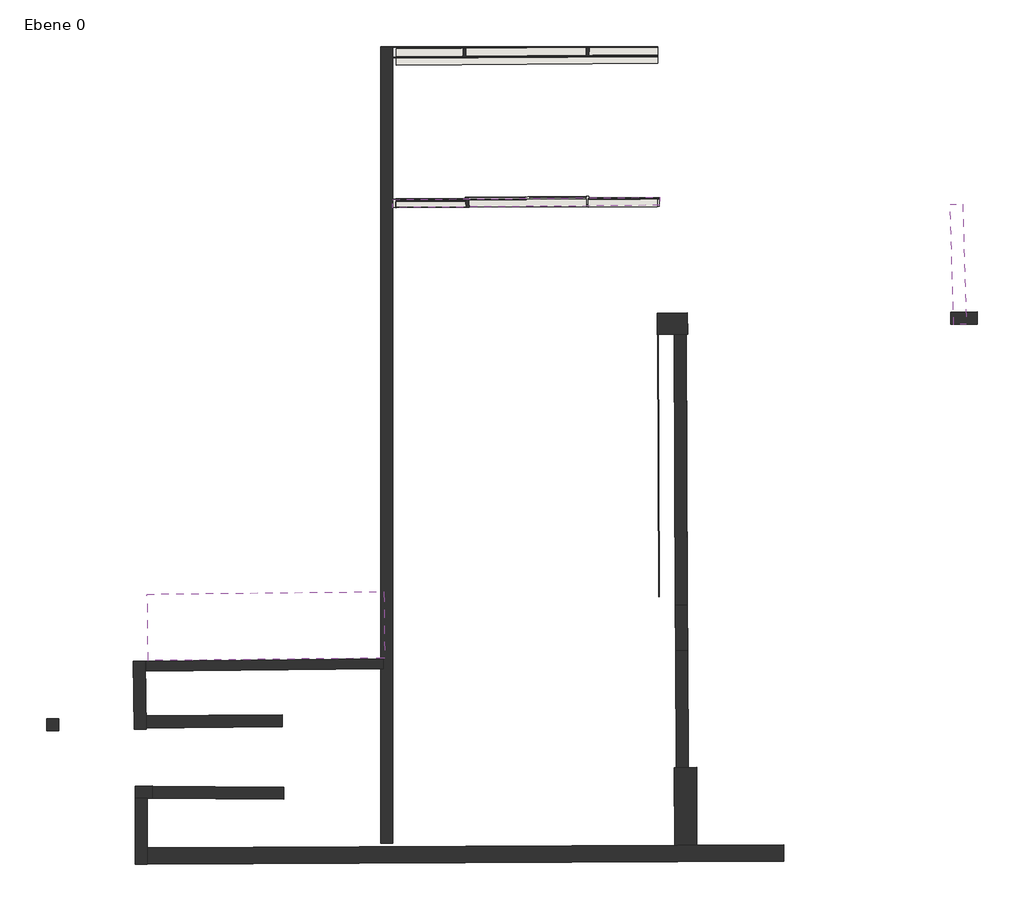
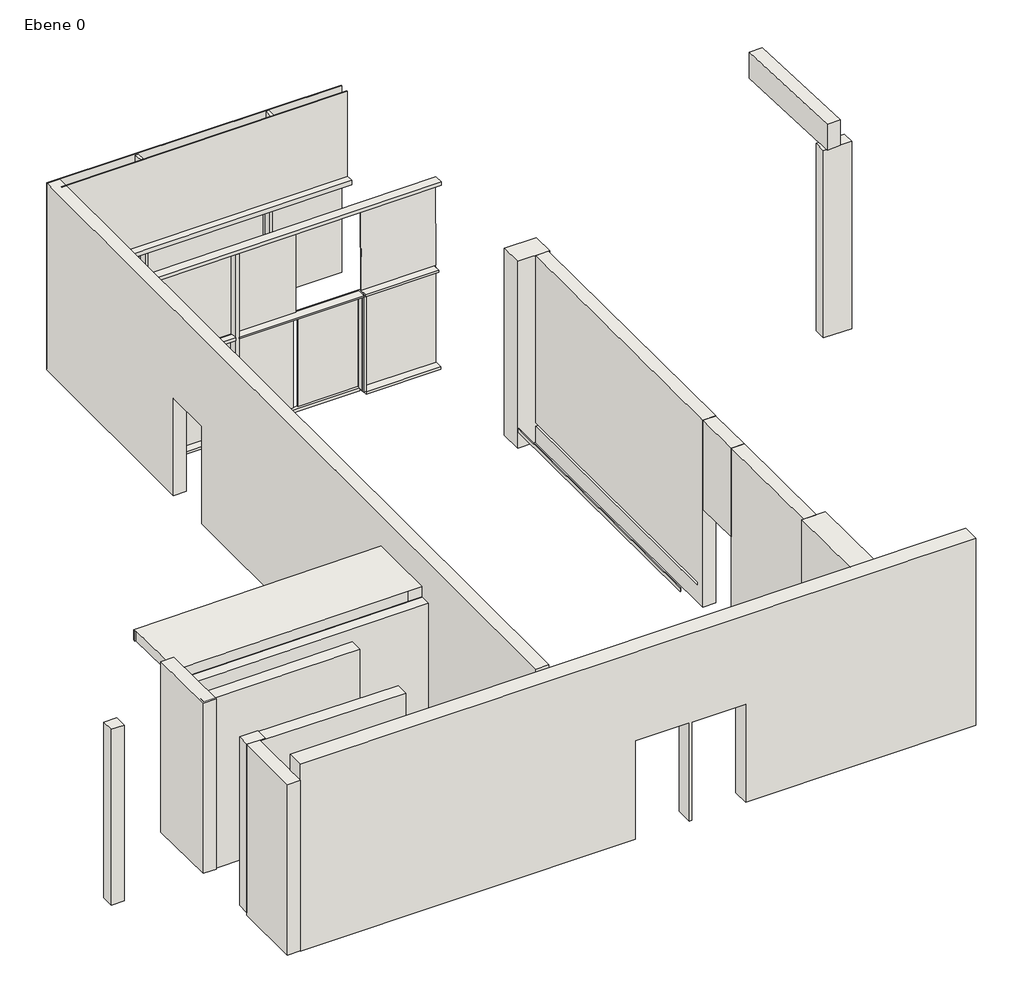
# One storey: 46 walls.
"""IFC4 building model written with IfcOpenShell, lengths in millimetres."""

from ifc_helpers import new_model, si_unit, frame, origin, place, context, project, spatial, polyline, outline, extrude, faceted_brep, element, save

model = new_model("IFC4")

# Units and contexts
model_context = context("Model", 3, world=origin())
ifc_project = project(units=[si_unit("LENGTHUNIT", "METRE", prefix="MILLI")], contexts=[model_context])

# Site, building, storey
site = spatial("IfcSite", under=ifc_project)
building = spatial("IfcBuilding", under=site)
storey = spatial("IfcBuildingStorey", under=building, Name="Ebene 0", Elevation=0.0)

# Walls
placement = place(None, origin())
element("IfcWall", 1, ObjectType="STB 30.0 - Sichtbeton 1", at=placement, inside=storey, context=model_context, shape_type="SweptSolid", body=[
    extrude(outline(polyline([(-8402.8984862, -3386.1116182), (-5023.0576004, -3407.986993), (-5024.9992525, -3707.9807096), (-8404.8401383, -3686.1053348), (-8402.8984862, -3386.1116182)])), frame((0.0, 0.0, -1567.0079424), z_axis=(0.0, 0.0, 1.0), x_axis=(1.0, 0.0, 0.0)), (0.0, 0.0, 1.0), 4193.9637451),
])
element("IfcWall", 2, ObjectType="STB 30.0 - Sichtbeton 1", at=placement, inside=storey, context=model_context, shape_type="SweptSolid", body=[
    extrude(outline(polyline([(-8711.881099, -1641.309095), (-5062.179794, -1608.676683), (-5059.4975656, -1908.6646922), (-8709.1988706, -1941.2971042), (-8711.881099, -1641.309095)])), frame((0.0, 0.0, -1566.6113359), z_axis=(0.0, 0.0, 1.0), x_axis=(1.0, 0.0, 0.0)), (0.0, 0.0, 1.0), 4193.494873),
])
element("IfcWall", 3, ObjectType="STB 30.0 - Sichtbeton 1", at=placement, inside=storey, context=model_context, shape_type="Brep", body=[
    faceted_brep([(-8280.7224922, -3375.8727385, -1505.4189133), (-8707.8712691, -3380.2933626, -1505.4189133), (-8707.8712691, -3380.2933626, 2636.550325), (-8280.7224922, -3375.8727385, 2636.550325), (-8280.7224922, -3375.8727385, -1388.9973215), (-8280.4523049, -3675.8860076, -1505.4189133), (-8280.4523049, -3675.8860076, 2636.550325), (-8407.8712691, -3677.2046848, 2636.550325), (-8707.8712691, -3680.3094278, 2636.550325), (-8707.8712691, -3680.3094278, -1505.4189133)], [[[0, 1, 2, 3, 4]], [[5, 6, 7, 8, 9]], [[1, 0, 5, 9]], [[3, 2, 8, 7, 6]], [[0, 4, 3, 6, 5]], [[2, 1, 9, 8]]]),
])
element("IfcWall", 4, ObjectType="STB 30.0 - Sichtbeton 1", at=placement, inside=storey, context=model_context, shape_type="Brep", body=[
    faceted_brep([(-8407.8712691, -5310.6242916, -1565.0), (-8407.8712691, -3677.2046848, -1565.0), (-8407.8712691, -3677.2046848, 2636.550325), (-8407.8712691, -5310.6242916, 2636.550325), (-8707.8712691, -5312.0476748, -1565.0), (-8707.8712691, -5312.0476748, 2636.550325), (-8707.8712691, -3680.3094278, 2636.550325), (-8707.8712691, -3680.3094278, -1505.4189133), (-8707.8712691, -3680.3094278, -1565.0)], [[[0, 1, 2, 3]], [[4, 5, 6, 7, 8]], [[1, 0, 4, 8]], [[3, 2, 6, 5]], [[2, 1, 8, 7, 6]], [[0, 3, 5, 4]]]),
])
element("IfcWall", 5, ObjectType="STB 30.0 - Sichtbeton 1", at=placement, inside=storey, context=model_context, shape_type="SweptSolid", body=[
    extrude(outline(polyline([(-8454.8872938, -283.8713377), (-8435.0535607, -1969.7388339), (-8735.0328016, -1973.268001), (-8754.8665347, -287.4005048), (-8454.8872938, -283.8713377)])), frame((0.0, 0.0, -1567.5369553), z_axis=(0.0, 0.0, 1.0), x_axis=(1.0, 0.0, 0.0)), (0.0, 0.0, 1.0), 4195.9727783),
])
element("IfcWall", 6, ObjectType="STB 30.0 - Sichtbeton 1", at=placement, inside=storey, context=model_context, shape_type="SweptSolid", body=[
    extrude(outline(polyline([(-10898.8481887, -2010.6735209), (-10902.7495019, -1710.7000992), (-10602.7748702, -1706.7987702), (-10598.873557, -2006.772192), (-10898.8481887, -2010.6735209)])), frame((0.0, 0.0, -1564.2386155), z_axis=(0.0, 0.0, 1.0), x_axis=(1.0, 0.0, 0.0)), (0.0, 0.0, 1.0), 4321.9161377),
])
element("IfcWall", 7, ObjectType="STB 30.0 - Sichtbeton 1", at=placement, inside=storey, context=model_context, shape_type="Brep", body=[
    faceted_brep([(4640.0905057, 7800.3536755, -1082.1717735), (4667.2831216, 1312.227188, -1082.1717735), (4667.2831216, 1312.227188, -1172.1717735), (4640.0905057, 7800.3536755, -1172.1717735), (4640.0905057, 7800.3536755, -1570.8115996), (4668.150891, 1105.1784267, -1570.8115996), (4668.150891, 1105.1784267, 3029.0079909), (4640.0905057, 7800.3536755, 3029.0079909), (4940.0878709, 7801.6110051, -1082.1717735), (4940.0878709, 7801.6110051, 3029.0079909), (4968.1456336, 1107.0614957, 3029.0079909), (4968.1456336, 1107.0614957, -1570.8115996), (4940.0878709, 7801.6110051, -1570.8115996), (4940.0878709, 7801.6110051, -1172.1717735), (4967.2804868, 1313.4845175, -1172.1717735), (4967.2804868, 1313.4845175, -1082.1717735)], [[[0, 1, 2, 3, 4, 5, 6, 7]], [[8, 9, 10, 11, 12, 13, 14, 15]], [[1, 0, 8, 15]], [[2, 1, 15, 14]], [[3, 2, 14, 13]], [[4, 3, 13, 12]], [[5, 4, 12, 11]], [[7, 6, 10, 9]], [[0, 7, 9, 8]], [[6, 5, 11, 10]]]),
])
element("IfcWall", 8, ObjectType="STB 30.0 - Sichtbeton 1", at=placement, inside=storey, context=model_context, shape_type="Brep", body=[
    faceted_brep([(4677.6567247, -31.4843616, 3026.055442), (4668.150891, 1105.1784267, 3026.055442), (4668.150891, 1105.1784267, 833.3), (4668.1769602, 1102.061196, 833.3), (4668.1769602, 1102.061196, 843.3), (4677.6567247, -31.4843616, 843.3), (4968.1456336, 1107.0614956, 3026.055442), (4977.6502256, -29.4528133, 3026.055442), (4977.6502256, -29.4528133, 843.3), (4968.1664699, 1104.5699879, 843.3), (4968.1664699, 1104.5699879, 833.3), (4968.1456336, 1107.0614956, 833.3)], [[[0, 1, 2, 3, 4, 5]], [[6, 7, 8, 9, 10, 11]], [[2, 11, 10, 3]], [[1, 0, 7, 6]], [[2, 1, 6, 11]], [[7, 0, 5, 8]], [[4, 9, 8, 5]], [[9, 4, 3, 10]]]),
])
element("IfcWall", 9, ObjectType="STB 30.0 - Sichtbeton 1", at=placement, inside=storey, context=model_context, shape_type="Brep", body=[
    faceted_brep([(4692.6152809, -2918.6509775, 3026.055442), (4677.6567247, -31.4843616, 3026.055442), (4677.6567247, -31.4843616, 843.3), (4677.6567247, -31.4843616, -1570.8115996), (4677.6744168, -34.8991368, -1570.8115996), (4692.6152809, -2918.6509775, -1570.8115996), (4992.6112545, -2917.0966832, 3026.055442), (4992.6112545, -2917.0966832, -1570.8115996), (4977.665445, -32.3903322, -1570.8115996), (4977.6502256, -29.4528134, -1570.8115996), (4977.6502256, -29.4528134, 843.3), (4977.6502256, -29.4528134, 3026.055442)], [[[0, 1, 2, 3, 4, 5]], [[6, 7, 8, 9, 10, 11]], [[1, 0, 6, 11]], [[5, 4, 3, 9, 8, 7]], [[0, 5, 7, 6]], [[3, 2, 1, 11, 10, 9]]]),
])
element("IfcWall", 10, ObjectType="STB 30.0 - Sichtbeton 1", at=placement, inside=storey, context=model_context, shape_type="Brep", body=[
    faceted_brep([(-2623.9258692, -4796.8405571, -1559.2743428), (-2623.9258692, -4796.8405571, 3034.8009859), (-2623.9258692, 14629.5579088, 3034.8009859), (-2623.9258692, 14919.5579088, 3034.8009859), (-2623.9258692, 14919.5579088, -1554.5282258), (-2623.9258692, 14939.5579088, -1554.5282258), (-2623.9258692, 14939.5579088, -1559.2743428), (-2623.9258692, 9821.2108055, -1559.2743428), (-2623.9258692, 9821.2108055, 843.3), (-2623.9258692, 8684.2108055, 843.3), (-2623.9258692, 8684.2108055, -1559.2743428), (-2623.9258692, 1234.2108055, -1559.2743428), (-2623.9258692, 1234.2108055, 843.3), (-2623.9258692, -25.7891945, 843.3), (-2623.9258692, -25.7891945, -1559.2743428), (-2323.9258692, -4796.8405571, 3034.8009859), (-2323.9258692, -4796.8405571, -1559.2743428), (-2323.9258692, -25.7891945, -1559.2743428), (-2323.9258692, -25.7891945, 843.3), (-2323.9258692, 1234.2108055, 843.3), (-2323.9258692, 1234.2108055, -1559.2743428), (-2323.9258692, 8684.2108055, -1559.2743428), (-2323.9258692, 8684.2108055, 843.3), (-2323.9258692, 9821.2108055, 843.3), (-2323.9258692, 9821.2108055, -1559.2743428), (-2323.9258692, 14939.5579088, -1559.2743428), (-2323.9258692, 14939.5579088, -1554.5282258), (-2323.9258692, 14919.5579088, -1554.5282258), (-2323.9258692, 14919.5579088, 3034.8009859), (-2473.9258692, 14919.5579088, 3034.8009859)], [[[0, 1, 2, 3, 4, 5, 6, 7, 8, 9, 10, 11, 12, 13, 14]], [[15, 16, 17, 18, 19, 20, 21, 22, 23, 24, 25, 26, 27, 28]], [[16, 0, 14, 17]], [[20, 11, 10, 21]], [[6, 25, 24, 7]], [[1, 0, 16, 15]], [[3, 2, 1, 15, 28, 29]], [[19, 12, 11, 20]], [[12, 19, 18, 13]], [[13, 18, 17, 14]], [[27, 26, 5, 4]], [[25, 6, 5, 26]], [[3, 29, 28, 27, 4]], [[23, 8, 7, 24]], [[8, 23, 22, 9]], [[9, 22, 21, 10]]]),
])
element("IfcWall", 11, ObjectType="STB 50.6 - Sichtbeton 9", at=placement, inside=storey, context=model_context, shape_type="Brep", body=[
    faceted_brep([(5199.7211413, -2916.1567546, 3026.055442), (5209.0004363, -4846.0130325, 3026.055442), (5209.0004363, -4846.0130325, -1564.9205192), (5199.7211413, -2916.1567546, -1571.9748716), (4649.727499, -2918.8012797, 3026.055442), (4649.727499, -2918.8012797, -1571.9748716), (4659.0066257, -4848.6225391, -1564.9206472), (4659.0066257, -4848.6225391, 3026.055442)], [[[0, 1, 2, 3]], [[4, 5, 6, 7]], [[1, 0, 4, 7]], [[3, 2, 6, 5]], [[0, 3, 5, 4]], [[2, 1, 7, 6]]]),
])
element("IfcWall", 12, ObjectType="STB 74.7 - Sichtbeton 8", at=placement, inside=storey, context=model_context, shape_type="SweptSolid", body=[
    extrude(outline(polyline([(4228.6457471, 7804.0053565), (4222.7195464, 8339.0935156), (4969.6737372, 8347.3661719), (4975.5999379, 7812.2780129), (4228.6457471, 7804.0053565)])), frame((0.0, 0.0, -1567.3220279), z_axis=(0.0, 0.0, 1.0), x_axis=(1.0, 0.0, 0.0)), (0.0, 0.0, 1.0), 4596.1280025),
])
element("IfcWall", 13, ObjectType="Sitzfläche Holz", at=placement, inside=storey, context=model_context, shape_type="SweptSolid", body=[
    extrude(outline(polyline([(4258.6670419, 1310.5146227), (4231.3829908, 7820.4574474), (4246.382859, 7820.5203138), (4273.6669102, 1310.5774892), (4258.6670419, 1310.5146227)])), frame((0.0, 0.0, -1172.1717735), z_axis=(0.0, 0.0, 1.0), x_axis=(1.0, 0.0, 0.0)), (0.0, 0.0, 1.0), 90.0),
])
element("IfcWall", 14, ObjectType="STB 30.0 - Sichtbeton 1", at=placement, inside=storey, context=model_context, shape_type="SweptSolid", body=[
    extrude(outline(polyline([(12156.2341991, 8065.3489209), (11495.6579868, 8063.6866533), (11494.9030721, 8363.6857035), (12156.2341991, 8365.3498707), (12156.2341991, 8065.3489209)])), frame((0.0, 0.0, -1554.8786442), z_axis=(0.0, 0.0, 1.0), x_axis=(1.0, 0.0, 0.0)), (0.0, 0.0, 1.0), 4605.4604069),
])
element("IfcWall", 15, ObjectType="STB 30.83 - Sichtbeton 10", at=placement, inside=storey, context=model_context, shape_type="SweptSolid", body=[
    extrude(outline(polyline([(11572.0416954, 8053.8502546), (11479.0551765, 11028.3975788), (11787.463897, 11029.737379), (11880.1911653, 8063.4832318), (11572.0416954, 8053.8502546)])), frame((0.0, 0.0, 3050.5817627), z_axis=(0.0, 0.0, 1.0), x_axis=(1.0, 0.0, 0.0)), (0.0, 0.0, 1.0), 634.2195252),
])
element("IfcWall", 16, ObjectType="Aluminiumrahmen 20cm", at=placement, inside=storey, context=model_context, shape_type="SweptSolid", body=[
    extrude(outline(polyline([(2530.9541861, 14704.8542909), (2466.9708915, 14706.1136197), (2470.9065593, 14906.0748922), (2534.889854, 14904.8155634), (2530.9541861, 14704.8542909)])), frame((0.0, 0.0, 963.2543258), z_axis=(0.0, 0.0, 1.0), x_axis=(1.0, 0.0, 0.0)), (0.0, 0.0, 1.0), 2077.8103027),
])
element("IfcWall", 17, ObjectType="Aluminiumrahmen 20cm", at=placement, inside=storey, context=model_context, shape_type="SweptSolid", body=[
    extrude(outline(polyline([(-516.6643868, 14688.191302), (-578.6088919, 14686.1559043), (-585.1770282, 14886.0480242), (-523.2325231, 14888.0834218), (-516.6643868, 14688.191302)])), frame((0.0, 0.0, 943.714653), z_axis=(0.0, 0.0, 1.0), x_axis=(1.0, 0.0, 0.0)), (0.0, 0.0, 1.0), 2096.5111084),
])
element("IfcWall", 18, ObjectType="Aluminiumrahmen 20cm", at=placement, inside=storey, context=model_context, shape_type="SweptSolid", body=[
    extrude(outline(polyline([(4241.1128382, 14525.186891), (-2240.5965186, 14482.3735992), (-2241.9175392, 14682.3692364), (4239.7918176, 14725.1825282), (4241.1128382, 14525.186891)])), frame((0.0, 0.0, 843.7151021), z_axis=(0.0, 0.0, 1.0), x_axis=(1.0, 0.0, 0.0)), (0.0, 0.0, 1.0), 99.9995509),
])
element("IfcWall", 19, ObjectType="Aluminiumrahmen 20cm", at=placement, inside=storey, context=model_context, shape_type="SweptSolid", body=[
    extrude(outline(polyline([(-454.8472123, 14616.4759781), (-496.8404301, 14616.0682776), (-498.7820831, 14816.0588524), (-456.7888653, 14816.4665529), (-454.8472123, 14616.4759781)])), frame((0.0, 0.0, -1569.2346878), z_axis=(0.0, 0.0, 1.0), x_axis=(1.0, 0.0, 0.0)), (0.0, 0.0, 1.0), 2407.9493408),
])
element("IfcWall", 20, ObjectType="Aluminiumrahmen 20cm", at=placement, inside=storey, context=model_context, shape_type="SweptSolid", body=[
    extrude(outline(polyline([(2451.6323777, 14636.0619156), (2403.6349929, 14636.4288193), (2405.163797, 14836.4229761), (2453.1611817, 14836.0560724), (2451.6323777, 14636.0619156)])), frame((0.0, 0.0, -1577.3386917), z_axis=(0.0, 0.0, 1.0), x_axis=(1.0, 0.0, 0.0)), (0.0, 0.0, 1.0), 2417.8755493),
])
element("IfcWall", 21, ObjectType="Aluminiumrahmen 20cm", at=placement, inside=storey, context=model_context, shape_type="SweptSolid", body=[
    extrude(outline(polyline([(-511.3662078, 10959.1183238), (-2319.8050257, 10959.1183238), (-2319.8050257, 11159.1183238), (-524.3930979, 11159.1183238), (-511.3662078, 10959.1183238)])), frame((0.0, 0.0, -1559.5502865), z_axis=(0.0, 0.0, 1.0), x_axis=(1.0, 0.0, 0.0)), (0.0, 0.0, 1.0), 51.7003161),
])
element("IfcWall", 22, ObjectType="Aluminiumrahmen 20cm 2", at=placement, inside=storey, context=model_context, shape_type="Brep", body=[
    faceted_brep([(-517.7933076, 11107.2777111, 900.0290089), (-517.9039135, 11105.9366786, 830.8928121), (-2250.633074, 11096.6298964, 833.8454007), (-2250.5224681, 11097.9709289, 902.9815975), (-2246.3874205, 11097.993139, 902.9745513), (-516.982536, 10957.2517121, 900.0290005), (-2245.5766498, 10947.96714, 902.9745429), (-2249.7116965, 10947.94493, 902.981589), (-2249.8223023, 10946.6038975, 833.8453923), (-517.0931419, 10955.9106796, 830.8928037)], [[[0, 1, 2, 3, 4]], [[5, 6, 7, 8, 9]], [[6, 5, 0, 4]], [[7, 6, 4, 3]], [[8, 7, 3, 2]], [[9, 8, 2, 1]], [[5, 9, 1, 0]]]),
])
element("IfcWall", 23, ObjectType="Aluminiumrahmen 20cm", at=placement, inside=storey, context=model_context, shape_type="SweptSolid", body=[
    extrude(outline(polyline([(2469.8899389, 10967.7043533), (-436.297192, 10960.4986908), (-449.3220187, 11160.4670115), (2469.3940561, 11167.7037385), (2469.8899389, 10967.7043533)])), frame((0.0, 0.0, 845.0347098), z_axis=(0.0, 0.0, 1.0), x_axis=(1.0, 0.0, 0.0)), (0.0, 0.0, 1.0), 43.8113839),
])
element("IfcWall", 24, ObjectType="Aluminiumrahmen 20cm", at=placement, inside=storey, context=model_context, shape_type="SweptSolid", body=[
    extrude(outline(polyline([(2532.2919931, 10975.5580245), (2470.5434806, 10975.7530127), (2471.1750336, 11175.7520156), (2532.9235461, 11175.5570273), (2532.2919931, 10975.5580245)])), frame((0.0, 0.0, -1500.4766489), z_axis=(0.0, 0.0, 1.0), x_axis=(1.0, 0.0, 0.0)), (0.0, 0.0, 1.0), 2345.5113587),
])
element("IfcWall", 25, ObjectType="Aluminiumrahmen 20cm", at=placement, inside=storey, context=model_context, shape_type="SweptSolid", body=[
    extrude(outline(polyline([(4289.3014273, 11005.4129185), (-2323.9258692, 10949.913032), (-2323.9258692, 11149.9200748), (4287.6230355, 11205.4058759), (4289.3014273, 11005.4129185)])), frame((0.0, 0.0, 2944.3505388), z_axis=(0.0, 0.0, 1.0), x_axis=(1.0, 0.0, 0.0)), (0.0, 0.0, 1.0), 86.6759664),
])
element("IfcWall", 26, ObjectType="Aluminiumrahmen 7,5cm", at=placement, inside=storey, context=model_context, shape_type="Brep", body=[
    faceted_brep([(-527.7117506, 11210.0691291, -1569.6072614), (-511.3662078, 10959.1183238, -1569.6072614), (-511.3662078, 10959.1183238, -1559.5502865), (-511.3662078, 10959.1183238, -1507.8499703), (-511.3662078, 10959.1183238, 2939.2424872), (-527.7117506, 11210.0691291, 2939.2424872), (-452.5886485, 11210.6191171, -1569.6072614), (-452.5886485, 11210.6191171, -1567.5099596), (-452.5886485, 11210.6191171, -1496.0611809), (-452.5886485, 11210.6191171, 2939.2424872), (-449.2570055, 11159.4688725, 2939.2424872), (-447.9543486, 11139.4693654, 2939.2424872), (-436.2072826, 10959.1183238, 2939.2424872), (-436.2072826, 10959.1183238, -1569.6072614)], [[[0, 1, 2, 3, 4, 5]], [[6, 7, 8, 9, 10, 11, 12, 13]], [[1, 0, 6, 13]], [[5, 4, 12, 11, 10, 9]], [[0, 5, 9, 8, 7, 6]], [[4, 3, 2, 1, 13, 12]]]),
])
element("IfcWall", 27, ObjectType="Aluminiumrahmen 20cm", at=placement, inside=storey, context=model_context, shape_type="SweptSolid", body=[
    extrude(outline(polyline([(4269.9303642, 10986.7075357), (2532.309784, 10981.1059862), (2531.6650494, 11181.104947), (4269.2856297, 11186.7064965), (4269.9303642, 10986.7075357)])), frame((0.0, 0.0, -1572.0237871), z_axis=(0.0, 0.0, 1.0), x_axis=(1.0, 0.0, 0.0)), (0.0, 0.0, 1.0), 62.3798925),
])
element("IfcWall", 28, ObjectType="Aluminiumrahmen 7,5cm", at=placement, inside=storey, context=model_context, shape_type="SweptSolid", body=[
    extrude(outline(polyline([(-452.5886485, 11210.6191171), (2478.4739757, 11232.0778854), (2479.0230477, 11157.0798953), (-447.7057623, 11135.6528555), (-452.5886485, 11210.6191171)])), frame((0.0, 0.0, -1567.5099596), z_axis=(0.0, 0.0, 1.0), x_axis=(1.0, 0.0, 0.0)), (0.0, 0.0, 1.0), 71.4487787),
])
element("IfcWall", 29, ObjectType="Aluminiumrahmen 20cm", at=placement, inside=storey, context=model_context, shape_type="SweptSolid", body=[
    extrude(outline(polyline([(2471.3474726, 11230.3596849), (2533.1410335, 11230.1645544), (2532.5094805, 11030.1655516), (2470.7159196, 11030.3606821), (2471.3474726, 11230.3596849)])), frame((0.0, 0.0, -1500.4766489), z_axis=(0.0, 0.0, 1.0), x_axis=(1.0, 0.0, 0.0)), (0.0, 0.0, 1.0), 2364.2643211),
])
element("IfcWall", 30, ObjectType="Aluminiumrahmen 20cm", at=placement, inside=storey, context=model_context, shape_type="SweptSolid", body=[
    extrude(outline(polyline([(4223.9186032, 10974.0579882), (2515.9054307, 10963.4053804), (2514.6580866, 11163.4014907), (4222.6712591, 11174.0540985), (4223.9186032, 10974.0579882)])), frame((0.0, 0.0, 845.0347098), z_axis=(0.0, 0.0, 1.0), x_axis=(1.0, 0.0, 0.0)), (0.0, 0.0, 1.0), 43.0983678),
])
element("IfcWall", 31, ObjectType="Aluminiumrahmen 20cm", at=placement, inside=storey, context=model_context, shape_type="SweptSolid", body=[
    extrude(outline(polyline([(-2243.2780557, 14888.3443346), (4238.4313012, 14931.1576264), (4239.7523218, 14731.1619892), (-2241.9570351, 14688.3486974), (-2243.2780557, 14888.3443346)])), frame((0.0, 0.0, 843.7151021), z_axis=(0.0, 0.0, 1.0), x_axis=(1.0, 0.0, 0.0)), (0.0, 0.0, 1.0), 99.9995509),
])
element("IfcWall", 32, ObjectType="Aluminiumrahmen 20cm", at=placement, inside=storey, context=model_context, shape_type="SweptSolid", body=[
    extrude(outline(polyline([(2405.7294156, 14910.4157336), (2453.7268003, 14910.0488299), (2452.1979963, 14710.0546731), (2404.2006116, 14710.4215768), (2405.7294156, 14910.4157336)])), frame((0.0, 0.0, -1577.3386917), z_axis=(0.0, 0.0, 1.0), x_axis=(1.0, 0.0, 0.0)), (0.0, 0.0, 1.0), 2417.8755493),
])
element("IfcWall", 33, ObjectType="Aluminiumrahmen 20cm", at=placement, inside=storey, context=model_context, shape_type="SweptSolid", body=[
    extrude(outline(polyline([(-499.4616302, 14886.0523207), (-457.4684125, 14886.4600212), (-455.5267595, 14686.4694465), (-497.5199772, 14686.0617459), (-499.4616302, 14886.0523207)])), frame((0.0, 0.0, -1569.2346878), z_axis=(0.0, 0.0, 1.0), x_axis=(1.0, 0.0, 0.0)), (0.0, 0.0, 1.0), 2407.9493408),
])
element("IfcWall", 34, ObjectType="Glasfassade", at=placement, inside=storey, context=model_context, shape_type="SweptSolid", body=[
    extrude(outline(polyline([(-449.2299687, 11212.4926831), (958.4892446, 11222.7988158), (958.6356638, 11202.7993518), (-449.0835495, 11192.4932191), (-449.2299687, 11212.4926831)])), frame((0.0, 0.0, -1496.0611809), z_axis=(0.0, 0.0, 1.0), x_axis=(1.0, 0.0, 0.0)), (0.0, 0.0, 1.0), 2344.345665),
])
element("IfcWall", 35, ObjectType="Glasfassade", at=placement, inside=storey, context=model_context, shape_type="SweptSolid", body=[
    extrude(outline(polyline([(1024.1639715, -19.9998824), (-1024.0267512, -19.9998823), (-1024.0953617, 0.0001177), (1024.095361, 0.0001177), (1024.1639715, -19.9998824)])), frame((-2241.2403215, 11125.2439305, 1920.2612034), z_axis=(0.9999647868922119, 0.00839195898543441, 0.0), x_axis=(-2.878865053450671e-05, 0.003430383399748157, 0.9999941158031603)), (0.0, 0.0, 1.0), 1723.3817094),
])
element("IfcWall", 36, ObjectType="Glasfassade", at=placement, inside=storey, context=model_context, shape_type="SweptSolid", body=[
    extrude(outline(polyline([(1028.3896086, -19.9987993), (-1027.9513066, -19.9987992), (-1028.1704708, 0.0012008), (1028.1704444, 0.0012008), (1028.3896086, -19.9987993)])), frame((2518.0878137, 11157.432084, 1916.2418082), z_axis=(0.999964786892212, 0.008391958985434413, 0.0), x_axis=(-9.195531599000662e-05, 0.010957164842832441, 0.9999399642392672)), (0.0, 0.0, 1.0), 1736.5032719),
])
element("IfcWall", 37, ObjectType="Glasfassade", at=placement, inside=storey, context=model_context, shape_type="SweptSolid", body=[
    extrude(outline(polyline([(4268.1486307, 11174.3377336), (2532.9787049, 11181.0998276), (2533.0566459, 11201.0996757), (4268.2265717, 11194.3375817), (4268.1486307, 11174.3377336)])), frame((0.0, 0.0, -1509.6438945), z_axis=(0.0, 0.0, 1.0), x_axis=(1.0, 0.0, 0.0)), (0.0, 0.0, 1.0), 2354.6786044),
])
element("IfcWall", 38, ObjectType="Glasfassade", at=placement, inside=storey, context=model_context, shape_type="SweptSolid", body=[
    extrude(outline(polyline([(-524.1136507, 11154.8280106), (-2249.5983951, 11147.9520531), (-2249.6780933, 11167.9518943), (-525.416012, 11174.8229795), (-524.1136507, 11154.8280106)])), frame((0.0, 0.0, -1507.8499703), z_axis=(0.0, 0.0, 1.0), x_axis=(1.0, 0.0, 0.0)), (0.0, 0.0, 1.0), 2334.8856416),
])
element("IfcWall", 39, ObjectType="Glasfassade", at=placement, inside=storey, context=model_context, shape_type="SweptSolid", body=[
    extrude(outline(polyline([(-449.2570055, 11159.4688725), (979.5144517, 11160.0111377), (979.5220423, 11140.0111392), (-447.9543486, 11139.4693654), (-449.2570055, 11159.4688725)])), frame((0.0, 0.0, 891.1173634), z_axis=(0.0, 0.0, 1.0), x_axis=(1.0, 0.0, 0.0)), (0.0, 0.0, 1.0), 2048.1251239),
])
element("IfcWall", 40, ObjectType="Glasfassade", at=placement, inside=storey, context=model_context, shape_type="SweptSolid", body=[
    extrude(outline(polyline([(1063.6949929, 11220.0540432), (2471.3474726, 11230.3596874), (2471.4938918, 11210.3602234), (1063.8414121, 11200.0545792), (1063.6949929, 11220.0540432)])), frame((0.0, 0.0, -1496.0611809), z_axis=(0.0, 0.0, 1.0), x_axis=(1.0, 0.0, 0.0)), (0.0, 0.0, 1.0), 2359.8488531),
])
element("IfcWall", 41, ObjectType="Glasfassade", at=placement, inside=storey, context=model_context, shape_type="SweptSolid", body=[
    extrude(outline(polyline([(1063.6949929, 11220.0540432), (2471.3474726, 11230.3596874), (2471.4938918, 11210.3602234), (1063.8414121, 11200.0545792), (1063.6949929, 11220.0540432)])), frame((0.0, 0.0, -1496.0611809), z_axis=(0.0, 0.0, 1.0), x_axis=(1.0, 0.0, 0.0)), (0.0, 0.0, 1.0), 2359.8488531),
])
element("IfcWall", 42, ObjectType="Glasfassade", at=placement, inside=storey, context=model_context, shape_type="Brep", body=[
    faceted_brep([(4235.0595919, 14919.5579088, -1554.5282258), (4235.0595919, 14919.5579088, 3035.7383094), (-2473.9258692, 14919.5579088, 3035.7383094), (-2473.9258692, 14919.5579088, 3034.8009859), (-2623.9258692, 14919.5579088, 3034.8009859), (-2623.9258692, 14919.5579088, -1554.5282258), (-2323.9258692, 14919.5579088, -1554.5282258), (4235.0595919, 14939.5579088, -1554.5282258), (-2323.9258692, 14939.5579088, -1554.5282258), (-2623.9258692, 14939.5579088, -1554.5282258), (-2623.9258692, 14939.5579088, 3034.8009859), (-2473.9258692, 14939.5579088, 3034.8009859), (-2473.9258692, 14939.5579088, 3035.7383094), (4235.0595919, 14939.5579088, 3035.7383094)], [[[0, 1, 2, 3, 4, 5, 6]], [[7, 8, 9, 10, 11, 12, 13]], [[1, 0, 7, 13]], [[2, 1, 13, 12]], [[0, 6, 5, 9, 8, 7]], [[3, 2, 12, 11]], [[3, 11, 10, 4]], [[5, 4, 10, 9]]]),
])
element("IfcWall", 43, ObjectType="Glasfassade", at=placement, inside=storey, context=model_context, shape_type="SweptSolid", body=[
    extrude(outline(polyline([(-2433.883637, 14669.1159954), (4236.984974, 14709.5666807), (4237.1062474, 14689.5670484), (-2433.7623637, 14649.116363), (-2433.883637, 14669.1159954)])), frame((0.0, 0.0, 894.7163796), z_axis=(0.0, 0.0, 1.0), x_axis=(1.0, 0.0, 0.0)), (0.0, 0.0, 1.0), 2140.7562727),
])
element("IfcWall", 44, ObjectType="STB 40.0 - Sichtbeton 7", at=placement, inside=storey, context=model_context, shape_type="Brep", body=[
    faceted_brep([(7358.7395645, -5235.8178592, -1577.6721536), (7358.7395645, -5235.8178592, 3028.7055287), (-8407.8712691, -5310.6242916, 3028.7055287), (-8407.8712691, -5310.6242916, 2636.550325), (-8407.8712691, -5310.6242916, -1565.0), (-8407.8712691, -5310.6242916, -1577.6721536), (-583.4447467, -5273.5004328, -1577.6721536), (-583.4447467, -5273.5004328, 843.3), (676.5410714, -5267.5222905, 843.3), (676.5410714, -5267.5222905, -1577.6721536), (726.8575404, -5267.2835584, -1577.6721536), (726.8575404, -5267.2835584, 843.3), (1986.8433585, -5261.3054161, 843.3), (1986.8433585, -5261.3054161, -1577.6721536), (7356.8417415, -4835.8223614, 3028.7055287), (7356.8417415, -4835.8223614, -1577.6721536), (1984.9455356, -4861.3099182, -1577.6721536), (1984.9455356, -4861.3099182, 843.3), (724.9597175, -4867.2880606, 843.3), (724.9597175, -4867.2880606, -1577.6721536), (674.6432484, -4867.5267927, -1577.6721536), (674.6432484, -4867.5267927, 843.3), (-585.3425697, -4873.504935, 843.3), (-585.3425697, -4873.504935, -1577.6721536), (-8407.8712691, -4910.6197893, -1577.6721536), (-8407.8712691, -4910.6197893, 3028.7055287)], [[[0, 1, 2, 3, 4, 5, 6, 7, 8, 9, 10, 11, 12, 13]], [[14, 15, 16, 17, 18, 19, 20, 21, 22, 23, 24, 25]], [[15, 0, 13, 16]], [[5, 24, 23, 6]], [[9, 20, 19, 10]], [[1, 0, 15, 14]], [[2, 1, 14, 25]], [[5, 4, 3, 2, 25, 24]], [[22, 7, 6, 23]], [[7, 22, 21, 8]], [[8, 21, 20, 9]], [[18, 11, 10, 19]], [[11, 18, 17, 12]], [[12, 17, 16, 13]]]),
])
element("IfcWall", 45, ObjectType="GK 25.0", at=placement, inside=storey, context=model_context, shape_type="SweptSolid", body=[
    extrude(outline(polyline([(0.0, 0.0), (3608.7078642, 0.0), (3608.6704113, -5888.6884598), (0.0266742, -5888.6884598), (0.0, 0.0)])), frame((-2563.8358921, -469.9186601, -1574.737862), z_axis=(-0.010857862877396351, 0.999941051669415, 0.0), x_axis=(0.0012161119308902936, 1.320515501101553e-05, 0.9999992604484242)), (0.0, 0.0, 1.0), 250.0),
])
element("IfcWall", 46, ObjectType="GK 25.0", at=placement, inside=storey, context=model_context, shape_type="SweptSolid", body=[
    extrude(outline(polyline([(-21540.6650721, 23920.4962764), (-26839.8897545, 21379.4135016), (-26859.1465615, 21419.6453465), (-27551.9062276, 22864.4135626), (-27174.8476023, 23045.1554225), (-22271.0517929, 25396.6222519), (-21577.9618072, 23952.0776279), (-21560.0463689, 23960.7073824), (-21540.6650721, 23920.4962764)])), frame((-17824.7416386, 32162.622769, 2048.895002), z_axis=(0.0012150993825128724, 0.00011277004424242195, 0.9999992554079268), x_axis=(-0.9061478884747843, 0.4229596844125457, 0.0010533633417530845)), (0.0, 0.0, 1.0), 250.0),
])

save(model, "model.ifc")

# Revit data of these elements
# Project information
#   Projektausgabedatum = "Projekt Datum"
#   Projektstatus = "Projektstatus"
#   Kundenname = "Bauherr"
#   Projektadresse = "Projektadresse"
#   Projektname = "Projektname"
#   Projektnummer = "Projektnummer"
#   Verfasser Firma 1 = "Firma 1"
#   Verfasser Firma 2 = "Firma 2"
#   Verfasser PLZ Ort = "PLZ Ort"
#   Verfasser Strasse = "Strasse"
#   Verfasser Telefon = "Telefon"
#   Verfasser Telefax = "Telefax"
#   Verfasser eMail = "E-Mail"
# Type "STB 30.0 - Sichtbeton 1"
#   Type Comments = "Stahlbeton Sichtbeton"
#   Description = "Stahlbeton (Sichtbeton) 30.0"
#   Layers, outside or top first: 0.300 m "Stahlbeton - Sichtbeton (1)" (function 1)
# Type "STB 50.6 - Sichtbeton 9"
#   Type Comments = "Stahlbeton Sichtbeton"
#   Description = "Stahlbeton (Sichtbeton) 30.0"
#   Layers, outside or top first: 0.550 m "Stahlbeton - Sichtbeton (1)" (function 1)
# Type "STB 74.7 - Sichtbeton 8"
#   Type Comments = "Stahlbeton Sichtbeton"
#   Description = "Stahlbeton (Sichtbeton) 30.0"
#   Layers, outside or top first: 0.747 m "Stahlbeton - Sichtbeton (1)" (function 1)
# Type "Sitzfläche Holz"
#   Type Comments = "Gipskarton"
#   Description = "1 x Gipskarton 1.25 cm, Metallständerprofil/Dämmung 7.5 cm, 1 x Gipskarton 1.25 cm"
#   Layers, outside or top first: 0.015 m "Holz - Birke" (function 2)
# Type "STB 30.83 - Sichtbeton 10"
#   Type Comments = "Stahlbeton Sichtbeton"
#   Description = "Stahlbeton (Sichtbeton) 30.0"
#   Layers, outside or top first: 0.3083 m "Stahlbeton - Sichtbeton (1)" (function 1)
# Type "Aluminiumrahmen 20cm"
#   Type Comments = "Standard"
#   Description = "Standardwand"
#   Layers, outside or top first: 0.200 m "Alumin." (function 1)
# Type "Aluminiumrahmen 20cm 2"
#   Type Comments = "Standard"
#   Description = "Standardwand"
#   Layers, outside or top first: 0.150 m "Alumin." (function 1)
# Type "Aluminiumrahmen 7,5cm"
#   Type Comments = "Standard"
#   Description = "Standardwand"
#   Layers, outside or top first: 0.075 m "Alumin." (function 1)
# Type "Glasfassade"
#   Type Comments = "Glasbaustein"
#   Description = "Glasbaustein 6.0 cm"
#   Layers, outside or top first: 0.020 m "Verglasung - Fensterverglasung" (function 1)
# Type "STB 40.0 - Sichtbeton 7"
#   Type Comments = "Stahlbeton Sichtbeton"
#   Description = "Stahlbeton (Sichtbeton) 30.0"
#   Layers, outside or top first: 0.400 m "Stahlbeton - Sichtbeton (1)" (function 1)
# Type "GK 25.0"
#   Type Comments = "Gipskarton"
#   Description = "2x Gipskarton 1.25 cm, Metallständerprofil/Dämmung 7.5 cm/ 5.0 cm/ 7.5 cm, 2x Gipskarton 1.25 cm"
#   Layers, outside or top first: 0.025 m "Gipswandbauplatte" (function 4); 0.075 m "Wärmedämmung - hart" (function 2); 0.050 m "Wärmedämmung - hart" (function 2); 0.075 m "Wärmedämmung - hart" (function 2); 0.025 m "Gipswandbauplatte" (function 5)
# Element 1 (IfcWall, "STB 30.0 - Sichtbeton 1")
#   built-in parameter 1001111 = -1.567008 m
#   Top Offset = 0.000 m
#   Base Offset = -1.567008 m
#   Unconnected Height = 4.193964 m
#   wall height = 4.193964 m
#   Phase Created = Phase 1
#   Base Constraint = Ebene 0
#   Materials on its faces: "Stahlbeton - Sichtbeton (1)"
# Element 2 (IfcWall, "STB 30.0 - Sichtbeton 1")
#   built-in parameter 1001111 = -1.566611 m
#   Top Offset = 0.000 m
#   Base Offset = -1.566611 m
#   Unconnected Height = 4.193495 m
#   wall height = 4.193495 m
#   Phase Created = Phase 1
#   Base Constraint = Ebene 0
#   Materials on its faces: "Stahlbeton - Sichtbeton (1)"
# Element 3 (IfcWall, "STB 30.0 - Sichtbeton 1")
#   built-in parameter 1001111 = -1.505419 m
#   Top Offset = 0.000 m
#   Base Offset = -1.505419 m
#   Unconnected Height = 4.141969 m
#   wall height = 4.141969 m
#   Phase Created = Phase 1
#   Base Constraint = Ebene 0
#   Materials on its faces: "Stahlbeton - Sichtbeton (1)"
# Element 4 (IfcWall, "STB 30.0 - Sichtbeton 1")
#   built-in parameter 1001111 = -1.565 m
#   Top Offset = 0.000 m
#   Base Offset = -1.565 m
#   Unconnected Height = 4.20155 m
#   wall height = 4.20155 m
#   Phase Created = Phase 1
#   Base Constraint = Ebene 0
#   Materials on its faces: "Stahlbeton - Sichtbeton (1)"
# Element 5 (IfcWall, "STB 30.0 - Sichtbeton 1")
#   built-in parameter 1001111 = -1.567537 m
#   Top Offset = 0.000 m
#   Base Offset = -1.567537 m
#   Unconnected Height = 4.195973 m
#   wall height = 4.195973 m
#   Phase Created = Phase 1
#   Base Constraint = Ebene 0
#   Materials on its faces: "Stahlbeton - Sichtbeton (1)"
# Element 6 (IfcWall, "STB 30.0 - Sichtbeton 1")
#   built-in parameter 1001111 = -1.564239 m
#   Top Offset = 0.000 m
#   Base Offset = -1.564239 m
#   Unconnected Height = 4.321916 m
#   wall height = 4.321916 m
#   Phase Created = Phase 1
#   Base Constraint = Ebene 0
#   Materials on its faces: "Stahlbeton - Sichtbeton (1)"
# Element 7 (IfcWall, "STB 30.0 - Sichtbeton 1")
#   built-in parameter 1001111 = -1.570812 m
#   Top Offset = 0.000 m
#   Base Offset = -1.570812 m
#   Unconnected Height = 4.59982 m
#   wall height = 4.59982 m
#   Phase Created = Phase 1
#   Base Constraint = Ebene 0
#   Materials on its faces: "Stahlbeton - Sichtbeton (1)"
# Element 8 (IfcWall, "STB 30.0 - Sichtbeton 1")
#   built-in parameter 1001111 = 0.8333 m
#   Top Offset = 0.000 m
#   Base Offset = 0.8333 m
#   Unconnected Height = 2.192755 m
#   wall height = 2.192755 m
#   Phase Created = Phase 1
#   Base Constraint = Ebene 0
#   Materials on its faces: "Stahlbeton - Sichtbeton (1)"
# Element 9 (IfcWall, "STB 30.0 - Sichtbeton 1")
#   built-in parameter 1001111 = -1.570812 m
#   Top Offset = 0.000 m
#   Base Offset = -1.570812 m
#   Unconnected Height = 4.596867 m
#   wall height = 4.596867 m
#   Phase Created = Phase 1
#   Base Constraint = Ebene 0
#   Materials on its faces: "Stahlbeton - Sichtbeton (1)"
# Element 10 (IfcWall, "STB 30.0 - Sichtbeton 1")
#   built-in parameter 1001111 = -1.559274 m
#   Top Offset = 0.000 m
#   Base Offset = -1.559274 m
#   Unconnected Height = 4.594075 m
#   wall height = 4.594075 m
#   Phase Created = Phase 1
#   Base Constraint = Ebene 0
#   Materials on its faces: "Stahlbeton - Sichtbeton (1)"
# Element 11 (IfcWall, "STB 50.6 - Sichtbeton 9")
#   built-in parameter 1001111 = -1.571975 m
#   Top Offset = 0.000 m
#   Base Offset = -1.571975 m
#   Unconnected Height = 4.59803 m
#   wall height = 4.59803 m
#   Phase Created = Phase 1
#   Base Constraint = Ebene 0
#   Materials on its faces: "Stahlbeton - Sichtbeton (1)"
# Element 12 (IfcWall, "STB 74.7 - Sichtbeton 8")
#   built-in parameter 1001111 = -1.567322 m
#   Top Offset = 0.000 m
#   Base Offset = -1.567322 m
#   Unconnected Height = 4.596128 m
#   wall height = 4.596128 m
#   Phase Created = Phase 1
#   Base Constraint = Ebene 0
#   Materials on its faces: "Stahlbeton - Sichtbeton (1)"
# Element 13 (IfcWall, "Sitzfläche Holz")
#   built-in parameter 1001111 = -1.172172 m
#   Top Offset = 0.000 m
#   Base Offset = -1.172172 m
#   Unconnected Height = 0.090 m
#   wall height = 0.090 m
#   Phase Created = Phase 1
#   Base Constraint = Ebene 0
#   Materials on its faces: "Holz - Birke"
# Element 14 (IfcWall, "STB 30.0 - Sichtbeton 1")
#   built-in parameter 1001111 = -1.554879 m
#   Top Offset = 0.000 m
#   Base Offset = -1.554879 m
#   Unconnected Height = 4.60546 m
#   wall height = 4.60546 m
#   Phase Created = Phase 1
#   Base Constraint = Ebene 0
#   Materials on its faces: "Stahlbeton - Sichtbeton (1)"
# Element 15 (IfcWall, "STB 30.83 - Sichtbeton 10")
#   built-in parameter 1001111 = 3.050582 m
#   Top Offset = 0.000 m
#   Base Offset = 3.050582 m
#   Unconnected Height = 0.63422 m
#   wall height = 0.63422 m
#   Phase Created = Phase 1
#   Base Constraint = Ebene 0
#   Materials on its faces: "Stahlbeton - Sichtbeton (1)"
# Element 16 (IfcWall, "Aluminiumrahmen 20cm")
#   built-in parameter 1001111 = 0.963254 m
#   Top Offset = 0.000 m
#   Base Offset = 0.963254 m
#   Unconnected Height = 2.07781 m
#   wall height = 2.07781 m
#   Phase Created = Phase 1
#   Base Constraint = Ebene 0
#   Materials on its faces: "Alumin."
# Element 17 (IfcWall, "Aluminiumrahmen 20cm")
#   built-in parameter 1001111 = 0.943715 m
#   Top Offset = 0.000 m
#   Base Offset = 0.943715 m
#   Unconnected Height = 2.096511 m
#   wall height = 2.096511 m
#   Phase Created = Phase 1
#   Base Constraint = Ebene 0
#   Materials on its faces: "Alumin."
# Elements 18, 31 (IfcWall, "Aluminiumrahmen 20cm")
#   built-in parameter 1001111 = 0.843715 m
#   Top Offset = 0.000 m
#   Base Offset = 0.843715 m
#   Unconnected Height = 0.100 m
#   wall height = 0.100 m
#   Phase Created = Phase 1
#   Base Constraint = Ebene 0
#   Materials on its faces: "Alumin."
# Elements 19, 33 (IfcWall, "Aluminiumrahmen 20cm")
#   built-in parameter 1001111 = -1.569235 m
#   Top Offset = 0.000 m
#   Base Offset = -1.569235 m
#   Unconnected Height = 2.407949 m
#   wall height = 2.407949 m
#   Phase Created = Phase 1
#   Base Constraint = Ebene 0
#   Materials on its faces: "Alumin."
# Elements 20, 32 (IfcWall, "Aluminiumrahmen 20cm")
#   built-in parameter 1001111 = -1.577339 m
#   Top Offset = 0.000 m
#   Base Offset = -1.577339 m
#   Unconnected Height = 2.417876 m
#   wall height = 2.417876 m
#   Phase Created = Phase 1
#   Base Constraint = Ebene 0
#   Materials on its faces: "Alumin."
# Element 21 (IfcWall, "Aluminiumrahmen 20cm")
#   built-in parameter 1001111 = -1.55955 m
#   Top Offset = 0.000 m
#   Base Offset = -1.55955 m
#   Unconnected Height = 0.0517 m
#   wall height = 0.0517 m
#   Phase Created = Phase 1
#   Base Constraint = Ebene 0
#   Materials on its faces: "Alumin."
# Element 22 (IfcWall, "Aluminiumrahmen 20cm 2")
#   Phase Created = Phase 1
#   Materials on its faces: "Alumin."
# Element 23 (IfcWall, "Aluminiumrahmen 20cm")
#   built-in parameter 1001111 = 0.845035 m
#   Top Offset = 0.000 m
#   Base Offset = 0.845035 m
#   Unconnected Height = 0.043811 m
#   wall height = 0.043811 m
#   Phase Created = Phase 1
#   Base Constraint = Ebene 0
#   Materials on its faces: "Alumin."
# Element 24 (IfcWall, "Aluminiumrahmen 20cm")
#   built-in parameter 1001111 = -1.500477 m
#   Top Offset = 0.000 m
#   Base Offset = -1.500477 m
#   Unconnected Height = 2.345511 m
#   wall height = 2.345511 m
#   Phase Created = Phase 1
#   Base Constraint = Ebene 0
#   Materials on its faces: "Alumin."
# Element 25 (IfcWall, "Aluminiumrahmen 20cm")
#   built-in parameter 1001111 = 2.944351 m
#   Top Offset = 0.000 m
#   Base Offset = 2.944351 m
#   Unconnected Height = 0.086676 m
#   wall height = 0.086676 m
#   Phase Created = Phase 1
#   Base Constraint = Ebene 0
#   Materials on its faces: "Alumin."
# Element 26 (IfcWall, "Aluminiumrahmen 7,5cm")
#   built-in parameter 1001111 = -1.569607 m
#   Top Offset = 0.000 m
#   Base Offset = -1.569607 m
#   Unconnected Height = 4.50885 m
#   wall height = 4.50885 m
#   Phase Created = Phase 1
#   Base Constraint = Ebene 0
#   Materials on its faces: "Alumin."
# Element 27 (IfcWall, "Aluminiumrahmen 20cm")
#   built-in parameter 1001111 = -1.572024 m
#   Top Offset = 0.000 m
#   Base Offset = -1.572024 m
#   Unconnected Height = 0.06238 m
#   wall height = 0.06238 m
#   Phase Created = Phase 1
#   Base Constraint = Ebene 0
#   Materials on its faces: "Alumin."
# Element 28 (IfcWall, "Aluminiumrahmen 7,5cm")
#   built-in parameter 1001111 = -1.56751 m
#   Top Offset = 0.000 m
#   Base Offset = -1.56751 m
#   Unconnected Height = 0.071449 m
#   wall height = 0.071449 m
#   Phase Created = Phase 1
#   Base Constraint = Ebene 0
#   Materials on its faces: "Alumin."
# Element 29 (IfcWall, "Aluminiumrahmen 20cm")
#   built-in parameter 1001111 = -1.500477 m
#   Top Offset = 0.000 m
#   Base Offset = -1.500477 m
#   Unconnected Height = 2.364264 m
#   wall height = 2.364264 m
#   Phase Created = Phase 1
#   Base Constraint = Ebene 0
#   Materials on its faces: "Alumin."
# Element 30 (IfcWall, "Aluminiumrahmen 20cm")
#   built-in parameter 1001111 = 0.845035 m
#   Top Offset = 0.000 m
#   Base Offset = 0.845035 m
#   Unconnected Height = 0.043098 m
#   wall height = 0.043098 m
#   Phase Created = Phase 1
#   Base Constraint = Ebene 0
#   Materials on its faces: "Alumin."
# Element 34 (IfcWall, "Glasfassade")
#   built-in parameter 1001111 = -1.496061 m
#   Top Offset = 0.000 m
#   Base Offset = -1.496061 m
#   Unconnected Height = 2.344346 m
#   wall height = 2.344346 m
#   Phase Created = Phase 1
#   Base Constraint = Ebene 0
#   Materials on its faces: "Verglasung - Fensterverglasung"
# Elements 35, 36 (IfcWall, "Glasfassade")
#   Phase Created = Phase 1
#   Materials on its faces: "Verglasung - Fensterverglasung"
# Element 37 (IfcWall, "Glasfassade")
#   built-in parameter 1001111 = -1.509644 m
#   Top Offset = 0.000 m
#   Base Offset = -1.509644 m
#   Unconnected Height = 2.354679 m
#   wall height = 2.354679 m
#   Phase Created = Phase 1
#   Base Constraint = Ebene 0
#   Materials on its faces: "Verglasung - Fensterverglasung"
# Element 38 (IfcWall, "Glasfassade")
#   built-in parameter 1001111 = -1.50785 m
#   Top Offset = 0.000 m
#   Base Offset = -1.50785 m
#   Unconnected Height = 2.334886 m
#   wall height = 2.334886 m
#   Phase Created = Phase 1
#   Base Constraint = Ebene 0
#   Materials on its faces: "Verglasung - Fensterverglasung"
# Element 39 (IfcWall, "Glasfassade")
#   built-in parameter 1001111 = 0.891117 m
#   Top Offset = 0.000 m
#   Base Offset = 0.891117 m
#   Unconnected Height = 2.048125 m
#   wall height = 2.048125 m
#   Phase Created = Phase 1
#   Base Constraint = Ebene 0
#   Materials on its faces: "Verglasung - Fensterverglasung"
# Elements 40, 41 (IfcWall, "Glasfassade")
#   built-in parameter 1001111 = -1.496061 m
#   Top Offset = 0.000 m
#   Base Offset = -1.496061 m
#   Unconnected Height = 2.359849 m
#   wall height = 2.359849 m
#   Phase Created = Phase 1
#   Base Constraint = Ebene 0
#   Materials on its faces: "Verglasung - Fensterverglasung"
# Element 42 (IfcWall, "Glasfassade")
#   built-in parameter 1001111 = -1.554528 m
#   Top Offset = 0.000 m
#   Base Offset = -1.554528 m
#   Unconnected Height = 4.590267 m
#   wall height = 4.590267 m
#   Phase Created = Phase 1
#   Base Constraint = Ebene 0
#   Materials on its faces: "Verglasung - Fensterverglasung", "Stahlbeton - Sichtbeton (1)"
# Element 43 (IfcWall, "Glasfassade")
#   built-in parameter 1001111 = 0.894716 m
#   Top Offset = 0.000 m
#   Base Offset = 0.894716 m
#   Unconnected Height = 2.140756 m
#   wall height = 2.140756 m
#   Phase Created = Phase 1
#   Base Constraint = Ebene 0
#   Materials on its faces: "Verglasung - Fensterverglasung"
# Element 44 (IfcWall, "STB 40.0 - Sichtbeton 7")
#   built-in parameter 1001111 = -1.577672 m
#   Top Offset = 0.000 m
#   Base Offset = -1.577672 m
#   Unconnected Height = 4.606378 m
#   wall height = 4.606378 m
#   Phase Created = Phase 1
#   Base Constraint = Ebene 0
#   Materials on its faces: "Stahlbeton - Sichtbeton (1)"
# Element 45 (IfcWall, "GK 25.0")
#   built-in parameter 1001111 = -1.575058 m
#   Top Offset = 0.000 m
#   Base Offset = -1.575058 m
#   Unconnected Height = 3.86614 m
#   wall height = 3.86614 m
#   Phase Created = Phase 1
#   Base Constraint = Ebene 0
#   Materials on its faces: "Gipswandbauplatte"
# Element 46 (IfcWall, "GK 25.0")
#   Phase Created = Phase 1
#   Materials on its faces: "Gipswandbauplatte"
# Materials
#   "Stahlbeton - Sichtbeton (1)": class "Beton", colour RGB 192 192 192, transparency 0, Cost = 0
#   "Holz - Birke": class "Holz", colour RGB 213 164 103, transparency 0, Cost = 0
#   "Alumin.": class "Metall", colour RGB 247 247 247, transparency 0, Description = "Aluminium 6061", Cost = 0
#   "Verglasung - Fensterverglasung": class "Glas", colour RGB 0 128 192, transparency 0.75, Description = "Klarglas", Cost = 0
#   "Gipswandbauplatte": class "Allgemeines", colour RGB 228 228 228, transparency 0, Description = "Gipswandbauplatte", Cost = 0
#   "Wärmedämmung - hart": class "Stuck", colour RGB 255 255 255, transparency 0, Description = "Äußere Oberfläche", Cost = 0
